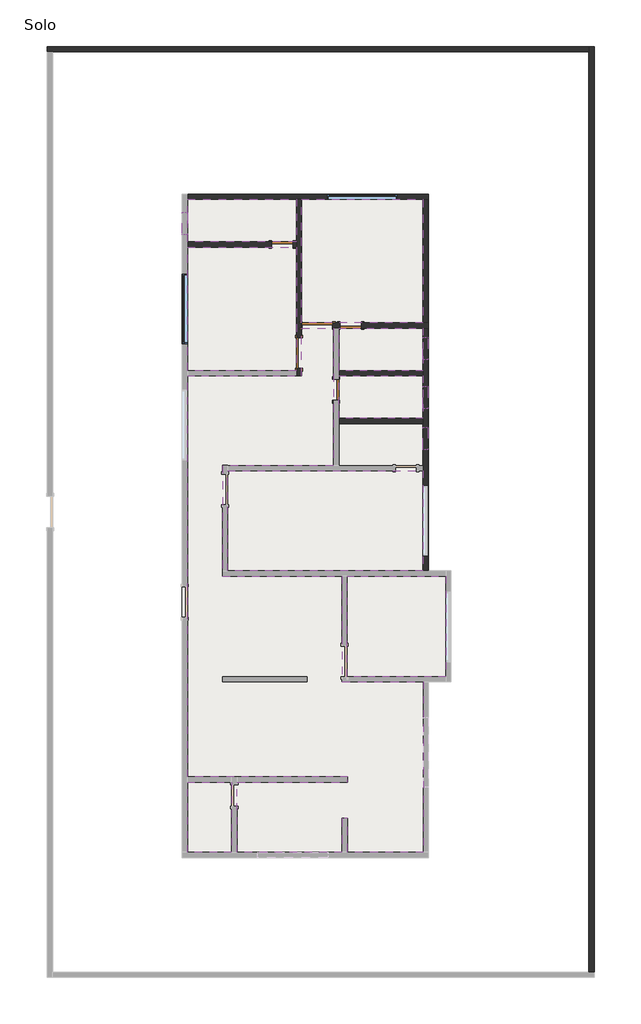
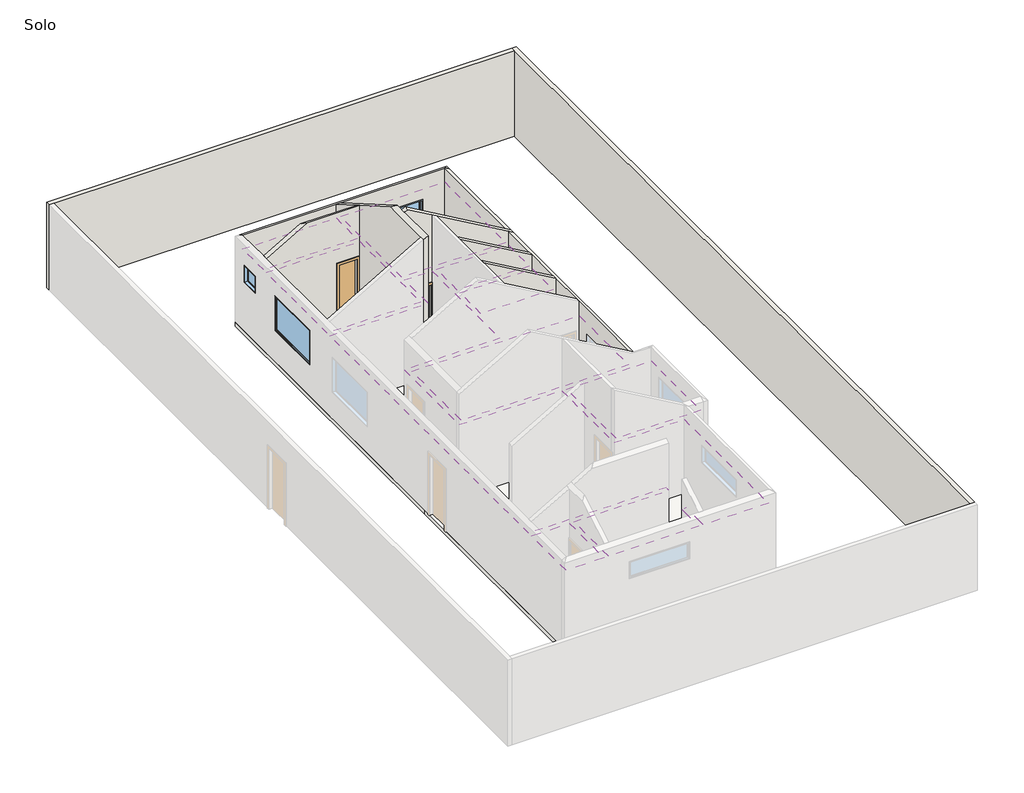
# One storey, part 2 of 2: 16 coverings, 9 walls, 6 windows, 5 doors, 1 slab.
"""IFC4 building model written with IfcOpenShell, lengths in millimetres."""

import ifcopenshell
import ifcopenshell.guid

model = None  # the IFC model being written
_history = None  # IfcOwnerHistory: only IFC2X3 demands one
_inside = {}  # id of a spatial element -> (the spatial element, [elements in it])
_under = {}  # id of a project, library or spatial element -> (it, [spatial elements below it])
_declared = {}  # id of a project -> (the project, [libraries it declares])
_typed = {}  # id of a type object -> (the type object, [elements of that type])
_made_of = {}  # id of a material, layer set ... -> (it, [elements and type objects made of it])


def new_model(schema):
    """Start an empty IFC model of exactly this schema.

    Asked for "IFC4X3", IfcOpenShell would pick the latest addendum, in which some entities
    have other attributes; the version numbers below select the first issue.
    IFC2X3 requires an IfcOwnerHistory on every rooted entity: one is made here for all.
    """
    global model, _history
    if schema == "IFC4X3":
        model = ifcopenshell.file(schema_version=(4, 3, 0, 0))
    else:
        model = ifcopenshell.file(schema=schema)
    _inside.clear()
    _under.clear()
    _declared.clear()
    _typed.clear()
    _made_of.clear()
    _history = None
    if model.schema == "IFC2X3":
        org = make("IfcOrganization", Name="unknown")
        user = make(
            "IfcPersonAndOrganization",
            ThePerson=make("IfcPerson", FamilyName="unknown"),
            TheOrganization=org,
        )
        app = make(
            "IfcApplication",
            ApplicationDeveloper=org,
            Version="unknown",
            ApplicationFullName="unknown",
            ApplicationIdentifier="unknown",
        )
        _history = make(
            "IfcOwnerHistory",
            OwningUser=user,
            OwningApplication=app,
            ChangeAction="ADDED",
            CreationDate=0,
        )
    return model


def make(cls, **values):
    """One entity of the class cls with the attributes given. An attribute that is None is left unset."""
    return model.create_entity(
        cls, **{name: value for name, value in values.items() if value is not None}
    )


def rooted(cls, **values):
    """An entity with a GlobalId (a new one), such as an element, a storey or a relation."""
    return make(cls, GlobalId=ifcopenshell.guid.new(), OwnerHistory=_history, **values)


def si_unit(unit_type, name, prefix=None):
    """IfcSIUnit, for example si_unit("LENGTHUNIT", "METRE", prefix="MILLI")."""
    return make("IfcSIUnit", UnitType=unit_type, Prefix=prefix, Name=name)


def assignment(units):
    """IfcUnitAssignment: the units of a project."""
    return None if units is None else make("IfcUnitAssignment", Units=units)


def point(xyz):
    """IfcCartesianPoint."""
    return None if xyz is None else make("IfcCartesianPoint", Coordinates=xyz)


def direction(xyz):
    """IfcDirection."""
    return None if xyz is None else make("IfcDirection", DirectionRatios=xyz)


def frame(location, z_axis=None, x_axis=None):
    """IfcAxis2Placement3D, a coordinate frame: its origin and axes. An axis left out is left unset."""
    return make(
        "IfcAxis2Placement3D",
        Location=point(location),
        Axis=direction(z_axis),
        RefDirection=direction(x_axis),
    )


def origin():
    """The frame at (0, 0, 0) with its axes left unset."""
    return frame((0.0, 0.0, 0.0))


def origin_with_axes():
    """The frame at (0, 0, 0) with the z axis (0, 0, 1) and the x axis (1, 0, 0) written out."""
    return frame((0.0, 0.0, 0.0), z_axis=(0.0, 0.0, 1.0), x_axis=(1.0, 0.0, 0.0))


def place(relative_to, where):
    """IfcLocalPlacement: puts the frame where relative to a parent placement (None: the world)."""
    return make(
        "IfcLocalPlacement", PlacementRelTo=relative_to, RelativePlacement=where
    )


def context(
    kind, dimensions, precision=None, world=None, true_north=None, identifier=None
):
    """IfcGeometricRepresentationContext, for example the 3D "Model" context."""
    return make(
        "IfcGeometricRepresentationContext",
        ContextIdentifier=identifier,
        ContextType=kind,
        CoordinateSpaceDimension=dimensions,
        Precision=precision,
        WorldCoordinateSystem=world,
        TrueNorth=true_north,
    )


def project(units=None, contexts=None):
    """IfcProject with its units and contexts."""
    return rooted(
        "IfcProject",
        Name="project",
        RepresentationContexts=contexts,
        UnitsInContext=assignment(units),
    )


def spatial(cls, under=None, at=None, **own):
    """A site, building, storey or space (cls), placed at a placement, below another one or the project."""
    s = rooted(cls, ObjectPlacement=at, **own)
    if under is not None:
        _under.setdefault(under.id(), (under, []))[1].append(s)
    return s


def polyline(points):
    """IfcPolyline through the points."""
    return make("IfcPolyline", Points=[point(p) for p in points])


def outline(outer, holes=None, kind="AREA"):
    """IfcArbitraryClosedProfileDef: a profile drawn as a closed curve; with holes, ...WithVoids."""
    if holes is None:
        return make("IfcArbitraryClosedProfileDef", ProfileType=kind, OuterCurve=outer)
    return make(
        "IfcArbitraryProfileDefWithVoids",
        ProfileType=kind,
        OuterCurve=outer,
        InnerCurves=holes,
    )


def extrude(swept, where, along, depth):
    """IfcExtrudedAreaSolid: the profile swept, set in the frame where, extruded along a direction by depth."""
    return make(
        "IfcExtrudedAreaSolid",
        SweptArea=swept,
        Position=where,
        ExtrudedDirection=direction(along),
        Depth=depth,
    )


def faces_of(points, faces, orient=None, outer=None):
    """IfcFace entities. A face is a list of loops; a loop is a list of indices into points, from 0.

    orient and outer hold one flag for each loop. By default every Orientation is true, the
    first loop of a face is its IfcFaceOuterBound and the others are IfcFaceBound.
    """
    made = []
    for i, loops in enumerate(faces):
        bounds = []
        for j, loop in enumerate(loops):
            is_outer = j == 0 if outer is None else outer[i][j]
            bounds.append(
                make(
                    "IfcFaceOuterBound" if is_outer else "IfcFaceBound",
                    Bound=make("IfcPolyLoop", Polygon=[points[k] for k in loop]),
                    Orientation=True if orient is None else orient[i][j],
                )
            )
        made.append(make("IfcFace", Bounds=bounds))
    return made


def faceted_brep(points, faces, orient=None, outer=None, voids=None):
    """IfcFacetedBrep: a solid bounded by flat faces; with voids (closed shells), ...WithVoids."""
    shared = [point(p) for p in points]
    hull = make("IfcClosedShell", CfsFaces=faces_of(shared, faces, orient, outer))
    if voids is None:
        return make("IfcFacetedBrep", Outer=hull)
    return make(
        "IfcFacetedBrepWithVoids",
        Outer=hull,
        Voids=[
            make(cls, CfsFaces=faces_of(shared, fs, o, b)) for cls, fs, o, b in voids
        ],
    )


def shape(context_of_items, identifier, shape_type, items):
    """IfcShapeRepresentation: the items that make up one representation, for example the "Body"."""
    return make(
        "IfcShapeRepresentation",
        ContextOfItems=context_of_items,
        RepresentationIdentifier=identifier,
        RepresentationType=shape_type,
        Items=items,
    )


def source(mapping_origin, context_of_items, identifier, shape_type, items):
    """IfcRepresentationMap: a shape defined once, which mapped items show again and again."""
    return make(
        "IfcRepresentationMap",
        MappingOrigin=mapping_origin,
        MappedRepresentation=shape(context_of_items, identifier, shape_type, items),
    )


def transform(
    local_origin,
    x_axis=None,
    y_axis=None,
    z_axis=None,
    scale=None,
    scale2=None,
    scale3=None,
    uniform=True,
):
    """IfcCartesianTransformationOperator3D, or its non-uniform kind. x_axis, y_axis, z_axis: its Axis1, 2, 3."""
    if uniform:
        return make(
            "IfcCartesianTransformationOperator3D",
            Axis1=direction(x_axis),
            Axis2=direction(y_axis),
            LocalOrigin=point(local_origin),
            Scale=scale,
            Axis3=direction(z_axis),
        )
    return make(
        "IfcCartesianTransformationOperator3DnonUniform",
        Axis1=direction(x_axis),
        Axis2=direction(y_axis),
        LocalOrigin=point(local_origin),
        Scale=scale,
        Axis3=direction(z_axis),
        Scale2=scale2,
        Scale3=scale3,
    )


def mapped(mapping_source, mapping_target):
    """IfcMappedItem: shows the shape of a source again, moved by a transform."""
    return make(
        "IfcMappedItem", MappingSource=mapping_source, MappingTarget=mapping_target
    )


def made_of(thing, what):
    """Note that an element or type object is made of a material, layer set ...; save() writes the relation."""
    if what is not None:
        _made_of.setdefault(what.id(), (what, []))[1].append(thing)
    return thing


def element(
    cls,
    number,
    at=None,
    inside=None,
    cuts=None,
    type_object=None,
    material=None,
    context=None,
    identifier="Body",
    shape_type=None,
    held_by="IfcProductDefinitionShape",
    body=None,
    shapes=None,
    **own,
):
    """One element of the class cls, such as IfcWall. Its Tag is "e" and its number.

    at: its placement. inside: the storey or other place that contains it. cuts: it is an
    opening in that element (IfcRelVoidsElement). A single representation is given by context,
    identifier, shape_type and body (its items); several are given by shapes. held_by: the class
    of the entity that holds the representations. save() writes the other relations.
    """
    e = rooted(cls, Tag="e%d" % number, ObjectPlacement=at, **own)
    if body is not None:
        shapes = [shape(context, identifier, shape_type, body)]
    if shapes is not None:
        e.Representation = make(held_by, Representations=shapes)
    if inside is not None:
        _inside.setdefault(inside.id(), (inside, []))[1].append(e)
    if cuts is not None:
        rooted(
            "IfcRelVoidsElement", RelatingBuildingElement=cuts, RelatedOpeningElement=e
        )
    if type_object is not None:
        _typed.setdefault(type_object.id(), (type_object, []))[1].append(e)
    return made_of(e, material)


def aggregate(whole, parts):
    """IfcRelAggregates: a whole, such as a stair, and the parts it consists of."""
    return rooted("IfcRelAggregates", RelatingObject=whole, RelatedObjects=parts)


def save(model, path):
    """Write the relations noted so far, then the file.

    IfcRelAggregates (storeys below a building ...), IfcRelContainedInSpatialStructure (elements
    in a storey), IfcRelDefinesByType, IfcRelAssociatesMaterial and IfcRelDeclares: one each for
    every whole, place, type object, material and project.
    """
    for whole, parts in _under.values():
        aggregate(whole, parts)
    for where, things in _inside.values():
        rooted(
            "IfcRelContainedInSpatialStructure",
            RelatedElements=things,
            RelatingStructure=where,
        )
    for kind, things in _typed.values():
        rooted("IfcRelDefinesByType", RelatedObjects=things, RelatingType=kind)
    for what, things in _made_of.values():
        rooted("IfcRelAssociatesMaterial", RelatedObjects=things, RelatingMaterial=what)
    for by, libraries in _declared.values():
        rooted("IfcRelDeclares", RelatingContext=by, RelatedDefinitions=libraries)
    model.write(path)


def door_0762_x_2032mm_f712f77f(model_context):
    return source(origin(), model_context, "Body", "SweptSolid", [
        extrude(outline(polyline([(2108.0, -376.0), (0.0, -376.0), (0.0, -300.0), (2032.0, -300.0), (2032.0, 300.0), (0.0, 300.0), (0.0, 376.0), (2108.0, 376.0), (2108.0, -376.0)])), frame((0.0, 75.0, 0.0), z_axis=(0.0, 1.0, 0.0), x_axis=(0.0, 0.0, 1.0)), (0.0, 0.0, 1.0), 25.0),
        extrude(outline(polyline([(2108.0, 376.0), (2108.0, -376.0), (0.0, -376.0), (0.0, -300.0), (2032.0, -300.0), (2032.0, 300.0), (0.0, 300.0), (0.0, 376.0), (2108.0, 376.0)])), frame((0.0, -100.0, 0.0), z_axis=(0.0, 1.0, 0.0), x_axis=(0.0, 0.0, 1.0)), (0.0, 0.0, 1.0), 25.0),
        extrude(outline(polyline([(300.0, 24.0), (-300.0, 24.0), (-300.0, 75.0), (300.0, 75.0), (300.0, 24.0)])), origin_with_axes(), (0.0, 0.0, 1.0), 2032.0),
    ])


def door_0762_x_2032mm_24b9c1ed(model_context):
    return source(origin(), model_context, "Body", "SweptSolid", [
        extrude(outline(polyline([(2108.0, -376.0), (0.0, -376.0), (0.0, -300.0), (2032.0, -300.0), (2032.0, 300.0), (0.0, 300.0), (0.0, 376.0), (2108.0, 376.0), (2108.0, -376.0)])), frame((0.0, -100.0, 0.0), z_axis=(0.0, 1.0, 0.0), x_axis=(0.0, 0.0, 1.0)), (0.0, 0.0, 1.0), 25.0),
        extrude(outline(polyline([(2108.0, 376.0), (2108.0, -376.0), (0.0, -376.0), (0.0, -300.0), (2032.0, -300.0), (2032.0, 300.0), (0.0, 300.0), (0.0, 376.0), (2108.0, 376.0)])), frame((0.0, 75.0, 0.0), z_axis=(0.0, 1.0, 0.0), x_axis=(0.0, 0.0, 1.0)), (0.0, 0.0, 1.0), 25.0),
        extrude(outline(polyline([(300.0, -24.0), (300.0, -75.0), (-300.0, -75.0), (-300.0, -24.0), (300.0, -24.0)])), origin_with_axes(), (0.0, 0.0, 1.0), 2032.0),
    ])


def door_0864_x_2134mm_0748c0c9(model_context):
    return source(origin(), model_context, "Body", "SweptSolid", [
        extrude(outline(polyline([(2210.0, -508.0), (0.0, -508.0), (0.0, -432.0), (2134.0, -432.0), (2134.0, 432.0), (0.0, 432.0), (0.0, 508.0), (2210.0, 508.0), (2210.0, -508.0)])), frame((0.0, -100.0, 0.0), z_axis=(0.0, 1.0, 0.0), x_axis=(0.0, 0.0, 1.0)), (0.0, 0.0, 1.0), 25.0),
        extrude(outline(polyline([(2210.0, 508.0), (2210.0, -508.0), (0.0, -508.0), (0.0, -432.0), (2134.0, -432.0), (2134.0, 432.0), (0.0, 432.0), (0.0, 508.0), (2210.0, 508.0)])), frame((0.0, 75.0, 0.0), z_axis=(0.0, 1.0, 0.0), x_axis=(0.0, 0.0, 1.0)), (0.0, 0.0, 1.0), 25.0),
        extrude(outline(polyline([(432.0, -24.0), (432.0, -75.0), (-432.0, -75.0), (-432.0, -24.0), (432.0, -24.0)])), origin_with_axes(), (0.0, 0.0, 1.0), 2134.0),
    ])


def m_fixo_0610_x_1830mm_9119c720(model_context):
    return source(origin(), model_context, "Body", "SweptSolid", [
        extrude(outline(polyline([(-257.0, 53.0), (257.0, 53.0), (257.0, 41.0), (-257.0, 41.0), (-257.0, 53.0)])), frame((0.0, 0.0, 668.0), z_axis=(0.0, 0.0, 1.0), x_axis=(1.0, 0.0, 0.0)), (0.0, 0.0, 1.0), 474.0),
        extrude(outline(polyline([(1186.0, -301.0), (624.0, -301.0), (624.0, 301.0), (1186.0, 301.0), (1186.0, -301.0)]), holes=[polyline([(1142.0, -257.0), (1142.0, 257.0), (668.0, 257.0), (668.0, -257.0), (1142.0, -257.0)])]), frame((0.0, 25.0, 0.0), z_axis=(0.0, 1.0, 0.0), x_axis=(0.0, 0.0, 1.0)), (0.0, 0.0, 1.0), 44.0),
        extrude(outline(polyline([(1205.0, -320.0), (605.0, -320.0), (605.0, 320.0), (1205.0, 320.0), (1205.0, -320.0)]), holes=[polyline([(1186.0, -301.0), (1186.0, 301.0), (624.0, 301.0), (624.0, -301.0), (1186.0, -301.0)])]), frame((0.0, 25.0, 0.0), z_axis=(0.0, 1.0, 0.0), x_axis=(0.0, 0.0, 1.0)), (0.0, 0.0, 1.0), 63.0),
        extrude(outline(polyline([(1205.0, -320.0), (605.0, -320.0), (605.0, 320.0), (1205.0, 320.0), (1205.0, -320.0)]), holes=[polyline([(1173.0, -288.0), (1173.0, 288.0), (637.0, 288.0), (637.0, -288.0), (1173.0, -288.0)])]), frame((0.0, -62.0, 0.0), z_axis=(0.0, 1.0, 0.0), x_axis=(0.0, 0.0, 1.0)), (0.0, 0.0, 1.0), 87.0),
    ])


def m_fixo_0915_x_1220mm_8e554ddc(model_context):
    return source(origin(), model_context, "Body", "SweptSolid", [
        extrude(outline(polyline([(-937.0, 53.0), (937.0, 53.0), (937.0, 41.0), (-937.0, 41.0), (-937.0, 53.0)])), frame((0.0, 0.0, 978.0), z_axis=(0.0, 0.0, 1.0), x_axis=(1.0, 0.0, 0.0)), (0.0, 0.0, 1.0), 1094.0),
        extrude(outline(polyline([(2116.0, -981.0), (934.0, -981.0), (934.0, 981.0), (2116.0, 981.0), (2116.0, -981.0)]), holes=[polyline([(2072.0, -937.0), (2072.0, 937.0), (978.0, 937.0), (978.0, -937.0), (2072.0, -937.0)])]), frame((0.0, 25.0, 0.0), z_axis=(0.0, 1.0, 0.0), x_axis=(0.0, 0.0, 1.0)), (0.0, 0.0, 1.0), 44.0),
        extrude(outline(polyline([(2135.0, -1000.0), (915.0, -1000.0), (915.0, 1000.0), (2135.0, 1000.0), (2135.0, -1000.0)]), holes=[polyline([(2116.0, -981.0), (2116.0, 981.0), (934.0, 981.0), (934.0, -981.0), (2116.0, -981.0)])]), frame((0.0, 25.0, 0.0), z_axis=(0.0, 1.0, 0.0), x_axis=(0.0, 0.0, 1.0)), (0.0, 0.0, 1.0), 63.0),
        extrude(outline(polyline([(2135.0, -1000.0), (915.0, -1000.0), (915.0, 1000.0), (2135.0, 1000.0), (2135.0, -1000.0)]), holes=[polyline([(2103.0, -968.0), (2103.0, 968.0), (947.0, 968.0), (947.0, -968.0), (2103.0, -968.0)])]), frame((0.0, -62.0, 0.0), z_axis=(0.0, 1.0, 0.0), x_axis=(0.0, 0.0, 1.0)), (0.0, 0.0, 1.0), 87.0),
    ])


model = new_model("IFC4")

# Units and contexts
model_context = context("Model", 3, world=origin())
ifc_project = project(units=[si_unit("LENGTHUNIT", "METRE", prefix="MILLI")], contexts=[model_context])

# Site, building, storey
site = spatial("IfcSite", under=ifc_project)
building = spatial("IfcBuilding", under=site)
storey = spatial("IfcBuildingStorey", under=building, Name="Solo", Elevation=0.0)

# Coverings
placement = place(None, origin())
element("IfcCovering", 1, ObjectType="Simples", at=placement, inside=storey, context=model_context, shape_type="SweptSolid", body=[
    extrude(outline(polyline([(-6285.8698767, 7725.0972586), (-6285.8698767, 8932.5972586), (-3187.4041224, 8932.5972586), (-3187.4041224, 7725.0972586), (-6285.8698767, 7725.0972586)])), frame((0.0, 0.0, 2600.0), z_axis=(0.0, 0.0, 1.0), x_axis=(1.0, 0.0, 0.0)), (0.0, 0.0, 1.0), 57.0),
])
element("IfcCovering", 2, ObjectType="Simples", at=placement, inside=storey, context=model_context, shape_type="SweptSolid", body=[
    extrude(outline(polyline([(-6285.8698767, 7725.0972586), (-6285.8698767, 8932.5972586), (-3187.4041224, 8932.5972586), (-3187.4041224, 7725.0972586), (-6285.8698767, 7725.0972586)])), frame((0.0, 0.0, 2600.0), z_axis=(0.0, 0.0, 1.0), x_axis=(1.0, 0.0, 0.0)), (0.0, 0.0, 1.0), 57.0),
])
element("IfcCovering", 3, ObjectType="Simples", at=placement, inside=storey, context=model_context, shape_type="SweptSolid", body=[
    extrude(outline(polyline([(-6285.8698767, 4070.0972586), (-6285.8698767, 7575.0972586), (-3187.4041224, 7575.0972586), (-3187.4041224, 4070.0972586), (-6285.8698767, 4070.0972586)])), frame((0.0, 0.0, 2600.0), z_axis=(0.0, 0.0, 1.0), x_axis=(1.0, 0.0, 0.0)), (0.0, 0.0, 1.0), 57.0),
])
element("IfcCovering", 4, ObjectType="Simples", at=placement, inside=storey, context=model_context, shape_type="SweptSolid", body=[
    extrude(outline(polyline([(-6285.8698767, 4070.0972586), (-6285.8698767, 7575.0972586), (-3187.4041224, 7575.0972586), (-3187.4041224, 4070.0972586), (-6285.8698767, 4070.0972586)])), frame((0.0, 0.0, 2600.0), z_axis=(0.0, 0.0, 1.0), x_axis=(1.0, 0.0, 0.0)), (0.0, 0.0, 1.0), 57.0),
])
element("IfcCovering", 5, ObjectType="Simples", at=placement, inside=storey, context=model_context, shape_type="SweptSolid", body=[
    extrude(outline(polyline([(-3037.4041224, 8932.5972586), (409.1301231, 8932.5972586), (409.1301231, 5423.5630139), (-3037.4041224, 5423.5630139), (-3037.4041224, 8932.5972586)])), frame((0.0, 0.0, 2600.0), z_axis=(0.0, 0.0, 1.0), x_axis=(1.0, 0.0, 0.0)), (0.0, 0.0, 1.0), 57.0),
])
element("IfcCovering", 6, ObjectType="Simples", at=placement, inside=storey, context=model_context, shape_type="SweptSolid", body=[
    extrude(outline(polyline([(-6285.8698767, 7725.0972586), (-6285.8698767, 8932.5972586), (-3187.4041224, 8932.5972586), (-3187.4041224, 7725.0972586), (-6285.8698767, 7725.0972586)])), frame((0.0, 0.0, 2600.0), z_axis=(0.0, 0.0, 1.0), x_axis=(1.0, 0.0, 0.0)), (0.0, 0.0, 1.0), 57.0),
])
element("IfcCovering", 7, ObjectType="Simples", at=placement, inside=storey, context=model_context, shape_type="SweptSolid", body=[
    extrude(outline(polyline([(-6285.8698767, 4070.0972586), (-6285.8698767, 7575.0972586), (-3187.4041224, 7575.0972586), (-3187.4041224, 4070.0972586), (-6285.8698767, 4070.0972586)])), frame((0.0, 0.0, 2600.0), z_axis=(0.0, 0.0, 1.0), x_axis=(1.0, 0.0, 0.0)), (0.0, 0.0, 1.0), 57.0),
])
element("IfcCovering", 8, ObjectType="Simples", at=placement, inside=storey, context=model_context, shape_type="SweptSolid", body=[
    extrude(outline(polyline([(-6285.8698767, 4070.0972586), (-6285.8698767, 7575.0972586), (-3187.4041224, 7575.0972586), (-3187.4041224, 4070.0972586), (-6285.8698767, 4070.0972586)])), frame((0.0, 0.0, 2600.0), z_axis=(0.0, 0.0, 1.0), x_axis=(1.0, 0.0, 0.0)), (0.0, 0.0, 1.0), 57.0),
])
element("IfcCovering", 9, ObjectType="Simples", at=placement, inside=storey, context=model_context, shape_type="SweptSolid", body=[
    extrude(outline(polyline([(-3037.4041224, 8932.5972586), (409.1301231, 8932.5972586), (409.1301231, 5423.5630139), (-3037.4041224, 5423.5630139), (-3037.4041224, 8932.5972586)])), frame((0.0, 0.0, 2600.0), z_axis=(0.0, 0.0, 1.0), x_axis=(1.0, 0.0, 0.0)), (0.0, 0.0, 1.0), 57.0),
])
element("IfcCovering", 10, ObjectType="Simples", at=placement, inside=storey, context=model_context, shape_type="SweptSolid", body=[
    extrude(outline(polyline([(-1979.4742231, 5273.5630139), (409.1301231, 5273.5630139), (409.1301231, 4070.0972586), (-1979.4742231, 4070.0972586), (-1979.4742231, 5273.5630139)])), frame((0.0, 0.0, 2600.0), z_axis=(0.0, 0.0, 1.0), x_axis=(1.0, 0.0, 0.0)), (0.0, 0.0, 1.0), 57.0),
])
element("IfcCovering", 11, ObjectType="Simples", at=placement, inside=storey, context=model_context, shape_type="SweptSolid", body=[
    extrude(outline(polyline([(409.1301231, 3920.0972586), (409.1301231, 2713.9475745), (-1979.4742231, 2713.9475745), (-1979.4742231, 3920.0972586), (409.1301231, 3920.0972586)])), frame((0.0, 0.0, 2600.0), z_axis=(0.0, 0.0, 1.0), x_axis=(1.0, 0.0, 0.0)), (0.0, 0.0, 1.0), 57.0),
])
element("IfcCovering", 12, ObjectType="Simples", at=placement, inside=storey, context=model_context, shape_type="SweptSolid", body=[
    extrude(outline(polyline([(424.1301232, -9623.7945276), (-1735.8698771, -9623.7945276), (-1735.8698771, -8644.9027402), (-1885.8698771, -8644.9027402), (-1885.8698771, -9623.7945276), (-4875.9149651, -9623.7945276), (-4875.9149651, -7626.6262329), (-1735.8698771, -7626.6262329), (-1735.8698771, -7476.6262329), (-4950.9149651, -7476.6262329), (-6285.8698767, -7476.6262329), (-6285.8698767, 3920.0972586), (-3037.4041224, 3920.0972586), (-3037.4041224, 5273.5630139), (-2129.4742231, 5273.5630139), (-2129.4742231, 1370.0972582), (-5289.335632, 1370.0972582), (-5289.335632, -1774.902741), (-1895.8247891, -1774.902741), (-1895.8247891, -4774.9027402), (424.1301232, -4774.9027402), (424.1301232, -9623.7945276)]), holes=[polyline([(-2885.8698771, -4774.9027402), (-2885.8698771, -4624.9027402), (-5285.8698771, -4624.9027402), (-5285.8698771, -4774.9027402), (-2885.8698771, -4774.9027402)])]), frame((0.0, 0.0, 2600.0), z_axis=(0.0, 0.0, 1.0), x_axis=(1.0, 0.0, 0.0)), (0.0, 0.0, 1.0), 57.0),
])
element("IfcCovering", 13, ObjectType="Simples", at=placement, inside=storey, context=model_context, shape_type="SweptSolid", body=[
    extrude(outline(polyline([(409.1301231, 1220.0972582), (409.1301231, -1624.902741), (-5139.335632, -1624.902741), (-5139.335632, 1220.0972582), (409.1301231, 1220.0972582)])), frame((0.0, 0.0, 2600.0), z_axis=(0.0, 0.0, 1.0), x_axis=(1.0, 0.0, 0.0)), (0.0, 0.0, 1.0), 57.0),
])
element("IfcCovering", 14, ObjectType="Simples", at=placement, inside=storey, context=model_context, shape_type="SweptSolid", body=[
    extrude(outline(polyline([(-1745.8247891, -1774.902741), (1059.1301231, -1774.902741), (1059.1301231, -4624.9027402), (-1745.8247891, -4624.9027402), (-1745.8247891, -1774.902741)])), frame((0.0, 0.0, 2600.0), z_axis=(0.0, 0.0, 1.0), x_axis=(1.0, 0.0, 0.0)), (0.0, 0.0, 1.0), 57.0),
])
element("IfcCovering", 15, ObjectType="Simples", at=placement, inside=storey, context=model_context, shape_type="SweptSolid", body=[
    extrude(outline(polyline([(424.1301232, -9623.7945276), (-1735.8698771, -9623.7945276), (-1735.8698771, -8644.9027402), (-1885.8698771, -8644.9027402), (-1885.8698771, -9623.7945276), (-4875.9149651, -9623.7945276), (-4875.9149651, -7626.6262329), (-1735.8698771, -7626.6262329), (-1735.8698771, -7476.6262329), (-4950.9149651, -7476.6262329), (-6285.8698767, -7476.6262329), (-6285.8698767, 3920.0972586), (-3037.4041224, 3920.0972586), (-3037.4041224, 5273.5630139), (-2129.4742231, 5273.5630139), (-2129.4742231, 1370.0972582), (-5289.335632, 1370.0972582), (-5289.335632, -1774.902741), (-1895.8247891, -1774.902741), (-1895.8247891, -4774.9027402), (424.1301232, -4774.9027402), (424.1301232, -9623.7945276)]), holes=[polyline([(-2885.8698771, -4774.9027402), (-2885.8698771, -4624.9027402), (-5285.8698771, -4624.9027402), (-5285.8698771, -4774.9027402), (-2885.8698771, -4774.9027402)])]), frame((0.0, 0.0, 2600.0), z_axis=(0.0, 0.0, 1.0), x_axis=(1.0, 0.0, 0.0)), (0.0, 0.0, 1.0), 57.0),
])
element("IfcCovering", 16, ObjectType="Simples", at=placement, inside=storey, context=model_context, shape_type="SweptSolid", body=[
    extrude(outline(polyline([(-5025.9149651, -9623.7945276), (-6285.8698767, -9623.7945276), (-6285.8698767, -7626.6262329), (-5025.9149651, -7626.6262329), (-5025.9149651, -9623.7945276)])), frame((0.0, 0.0, 2600.0), z_axis=(0.0, 0.0, 1.0), x_axis=(1.0, 0.0, 0.0)), (0.0, 0.0, 1.0), 57.0),
])

# Doors
door_0762_x_2032mm_shape = door_0762_x_2032mm_f712f77f(model_context)
element("IfcDoor", 17, ObjectType="M_Folha única : 0762 x 2032mm", at=placement, inside=storey, context=model_context, shape_type="MappedRepresentation", body=[
    mapped(door_0762_x_2032mm_shape, transform((-3587.4041224, 7650.0972586, 0.0), x_axis=(1.0, 0.0, 0.0), y_axis=(0.0, 1.0, 0.0), z_axis=(0.0, 0.0, 1.0))),
])
element("IfcDoor", 18, ObjectType="M_Folha única : 0762 x 2032mm", at=placement, inside=storey, context=model_context, shape_type="MappedRepresentation", body=[
    mapped(door_0762_x_2032mm_shape, transform((-1639.4742231, 5348.5630139, 0.0), x_axis=(-1.0, 0.0, 0.0), y_axis=(0.0, -1.0, 0.0), z_axis=(0.0, 0.0, 1.0))),
])
door_0762_x_2032mm_2_shape = door_0762_x_2032mm_24b9c1ed(model_context)
element("IfcDoor", 19, ObjectType="M_Folha única : 0762 x 2032mm", at=placement, inside=storey, context=model_context, shape_type="MappedRepresentation", body=[
    mapped(door_0762_x_2032mm_2_shape, transform((-2054.4742231, 3520.0972586, 0.0), x_axis=(0.0, 1.0, 0.0), y_axis=(-1.0, 0.0, 0.0), z_axis=(0.0, 0.0, 1.0))),
])
door_0864_x_2134mm_shape = door_0864_x_2134mm_0748c0c9(model_context)
element("IfcDoor", 20, ObjectType="M_Folha única : 0864 x 2134mm", at=placement, inside=storey, context=model_context, shape_type="MappedRepresentation", body=[
    mapped(door_0864_x_2134mm_shape, transform((-3112.4041224, 4562.0972586, 0.0), x_axis=(0.0, -1.0, 0.0), y_axis=(1.0, 0.0, 0.0), z_axis=(0.0, 0.0, 1.0))),
])
element("IfcDoor", 21, ObjectType="M_Folha única : 0864 x 2134mm", at=placement, inside=storey, context=model_context, shape_type="MappedRepresentation", body=[
    mapped(door_0864_x_2134mm_shape, transform((-2586.5671697, 5348.5630139, 0.0), x_axis=(-1.0, 0.0, 0.0), y_axis=(0.0, -1.0, 0.0), z_axis=(0.0, 0.0, 1.0))),
])

# Slab
element("IfcSlab", 22, ObjectType="Genérico 150 mm", at=placement, inside=storey, context=model_context, shape_type="SweptSolid", body=[
    extrude(outline(polyline([(-6435.8698767, 9082.5972586), (574.1301232, 9082.5972586), (574.1301232, -1624.902741), (1209.1301231, -1624.902741), (1209.1301231, -4774.9027402), (574.1301232, -4774.9027402), (574.1301232, -9773.7945276), (-6435.8698767, -9773.7945276), (-6435.8698767, -1774.902741), (-6435.8698767, 9082.5972586)])), frame((0.0, 0.0, -150.0), z_axis=(0.0, 0.0, 1.0), x_axis=(1.0, 0.0, 0.0)), (0.0, 0.0, 1.0), 150.0),
])

# Walls
element("IfcWall", 23, ObjectType="Genérico - 140 mm Alvenaria", at=placement, inside=storey, context=model_context, shape_type="Brep", body=[
    faceted_brep([(564.1301231, 9082.5972586, 0.0), (-6285.8698767, 9082.5972586, 0.0), (-6285.8698767, 9082.5972586, 3000.0), (564.1301231, 9082.5972586, 3000.0), (-2314.1369996, 9082.5972586, 1021.335877), (-314.1369996, 9082.5972586, 1021.335877), (-314.1369996, 9082.5972586, 2241.335877), (-2314.1369996, 9082.5972586, 2241.335877), (564.1301231, 8932.5972586, 0.0), (564.1301231, 8932.5972586, 3005.7735027), (559.1301231, 8932.5972586, 3008.6602541), (424.1301232, 8932.5972586, 3086.6025404), (409.1301231, 8932.5972586, 3086.6025404), (-3037.4041224, 8932.5972586, 3086.6025404), (-3187.4041224, 8932.5972586, 3086.6025404), (-6285.8698767, 8932.5972586, 3086.6025404), (-6285.8698767, 8932.5972586, 0.0), (-3187.4041224, 8932.5972586, 0.0), (-3037.4041224, 8932.5972586, 0.0), (409.1301231, 8932.5972586, 0.0), (559.1301231, 8932.5972586, 0.0), (-2314.1369996, 8932.5972586, 1021.335877), (-2314.1369996, 8932.5972586, 2241.335877), (-314.1369996, 8932.5972586, 2241.335877), (-314.1369996, 8932.5972586, 1021.335877), (564.1301231, 9072.5972586, 3005.7735027)], [[[0, 1, 2, 3], [4, 5, 6, 7]], [[8, 9, 10, 11, 12, 13, 14, 15, 16, 17, 18, 19, 20], [21, 22, 23, 24]], [[1, 0, 8, 20, 19, 18, 17, 16]], [[0, 3, 25, 9, 8]], [[2, 1, 16, 15]], [[22, 21, 4, 7]], [[23, 22, 7, 6]], [[24, 23, 6, 5]], [[21, 24, 5, 4]], [[3, 2, 15, 14, 13, 12, 11, 25]], [[11, 10, 9, 25]]]),
])
element("IfcWall", 24, ObjectType="Genérico - 140 mm Alvenaria", at=placement, inside=storey, context=model_context, shape_type="Brep", body=[
    faceted_brep([(-3187.4041224, 7725.0972586, 0.0), (-3287.4041224, 7725.0972586, 0.0), (-3287.4041224, 7725.0972586, 2032.0), (-3887.4041224, 7725.0972586, 2032.0), (-3887.4041224, 7725.0972586, 0.0), (-6285.8698767, 7725.0972586, 0.0), (-6285.8698767, 7725.0972586, 3086.6025404), (-5078.3698767, 7725.0972586, 3783.7529904), (-3187.4041224, 7725.0972586, 3783.7529904), (-3287.4041224, 7575.0972586, 2032.0), (-3287.4041224, 7575.0972586, 0.0), (-3187.4041224, 7575.0972586, 0.0), (-3187.4041224, 7575.0972586, 3870.3555308), (-4928.3698767, 7575.0972586, 3870.3555308), (-6285.8698767, 7575.0972586, 3086.6025404), (-6285.8698767, 7575.0972586, 0.0), (-3887.4041224, 7575.0972586, 0.0), (-3887.4041224, 7575.0972586, 2032.0)], [[[0, 1, 2, 3, 4, 5, 6, 7, 8]], [[9, 10, 11, 12, 13, 14, 15, 16, 17]], [[16, 15, 5, 4]], [[11, 10, 1, 0]], [[6, 5, 15, 14]], [[0, 8, 12, 11]], [[2, 1, 10, 9]], [[3, 2, 9, 17]], [[4, 3, 17, 16]], [[8, 7, 13, 12]], [[7, 6, 14, 13]]]),
])
element("IfcWall", 25, ObjectType="Genérico - 140 mm Alvenaria", at=placement, inside=storey, context=model_context, shape_type="Brep", body=[
    faceted_brep([(-3037.4041224, 3920.0972586, 0.0), (-3037.4041224, 4130.0972586, 0.0), (-3037.4041224, 4130.0972586, 2134.0), (-3037.4041224, 4994.0972586, 2134.0), (-3037.4041224, 4994.0972586, 0.0), (-3037.4041224, 5273.5630139, 0.0), (-3037.4041224, 5423.5630139, 0.0), (-3037.4041224, 8932.5972586, 0.0), (-3037.4041224, 8932.5972586, 3086.6025404), (-3037.4041224, 5684.1315043, 4962.1051181), (-3037.4041224, 5423.5630139, 4962.1051181), (-3037.4041224, 5273.5630139, 4962.1051181), (-3037.4041224, 3920.0972586, 4962.1051181), (-3187.4041224, 4130.0972586, 2134.0), (-3187.4041224, 4130.0972586, 0.0), (-3187.4041224, 4070.0972586, 0.0), (-3187.4041224, 3920.0972586, 0.0), (-3187.4041224, 3920.0972586, 4875.5025777), (-3187.4041224, 4070.0972586, 4875.5025777), (-3187.4041224, 5834.1315043, 4875.5025777), (-3187.4041224, 7575.0972586, 3870.3555308), (-3187.4041224, 7725.0972586, 3783.7529904), (-3187.4041224, 8932.5972586, 3086.6025404), (-3187.4041224, 8932.5972586, 0.0), (-3187.4041224, 7725.0972586, 0.0), (-3187.4041224, 7575.0972586, 0.0), (-3187.4041224, 4994.0972586, 0.0), (-3187.4041224, 4994.0972586, 2134.0)], [[[0, 1, 2, 3, 4, 5, 6, 7, 8, 9, 10, 11, 12]], [[13, 14, 15, 16, 17, 18, 19, 20, 21, 22, 23, 24, 25, 26, 27]], [[16, 15, 14, 1, 0]], [[26, 25, 24, 23, 7, 6, 5, 4]], [[8, 7, 23, 22]], [[0, 12, 17, 16]], [[2, 1, 14, 13]], [[3, 2, 13, 27]], [[4, 3, 27, 26]], [[12, 11, 10, 9, 19, 18, 17]], [[9, 8, 22, 21, 20, 19]]]),
])
element("IfcWall", 26, ObjectType="Genérico - 140 mm Alvenaria", at=placement, inside=storey, context=model_context, shape_type="Brep", body=[
    faceted_brep([(-1939.4742231, 5423.5630139, 2032.0), (-1939.4742231, 5423.5630139, 0.0), (-2154.5671697, 5423.5630139, 0.0), (-2154.5671697, 5423.5630139, 2134.0), (-3018.5671697, 5423.5630139, 2134.0), (-3018.5671697, 5423.5630139, 0.0), (-3037.4041224, 5423.5630139, 0.0), (-3037.4041224, 5423.5630139, 4962.1051181), (-2930.8698768, 5423.5630139, 5023.6126935), (564.1301231, 5423.5630139, 3005.7735027), (564.1301231, 5423.5630139, 0.0), (-1339.4742231, 5423.5630139, 0.0), (-1339.4742231, 5423.5630139, 2032.0), (-2154.5671697, 5273.5630139, 0.0), (-2129.4742231, 5273.5630139, 0.0), (-1979.4742231, 5273.5630139, 0.0), (-1939.4742231, 5273.5630139, 0.0), (-1939.4742231, 5273.5630139, 2032.0), (-1339.4742231, 5273.5630139, 2032.0), (-1339.4742231, 5273.5630139, 0.0), (564.1301231, 5273.5630139, 0.0), (564.1301231, 5273.5630139, 3005.7735027), (-1979.4742231, 5273.5630139, 4474.3241567), (-2129.4742231, 5273.5630139, 4560.9266971), (-2930.8698768, 5273.5630139, 5023.6126935), (-3037.4041224, 5273.5630139, 4962.1051181), (-3037.4041224, 5273.5630139, 0.0), (-3018.5671697, 5273.5630139, 0.0), (-3018.5671697, 5273.5630139, 2134.0), (-2154.5671697, 5273.5630139, 2134.0)], [[[0, 1, 2, 3, 4, 5, 6, 7, 8, 9, 10, 11, 12]], [[13, 14, 15, 16, 17, 18, 19, 20, 21, 22, 23, 24, 25, 26, 27, 28, 29]], [[6, 5, 27, 26]], [[11, 10, 20, 19]], [[2, 1, 16, 15, 14, 13]], [[10, 9, 21, 20]], [[7, 6, 26, 25]], [[28, 27, 5, 4]], [[29, 28, 4, 3]], [[13, 29, 3, 2]], [[17, 16, 1, 0]], [[18, 17, 0, 12]], [[19, 18, 12, 11]], [[9, 8, 24, 23, 22, 21]], [[8, 7, 25, 24]]]),
])
element("IfcWall", 27, ObjectType="Genérico - 140 mm Alvenaria", at=placement, inside=storey, context=model_context, shape_type="Brep", body=[
    faceted_brep([(409.1301231, 8932.5972586, 0.0), (409.1301231, 4070.0972586, 0.0), (409.1301231, 3920.0972586, 0.0), (409.1301231, 2713.9475745, 0.0), (409.1301231, 2563.9475745, 0.0), (409.1301231, 1370.0972582, 0.0), (409.1301231, 1220.0972582, 0.0), (409.1301231, -1624.902741, 0.0), (409.1301231, -1624.902741, 3095.2627944), (409.1301231, 1220.0972582, 3095.2627944), (409.1301231, 1370.0972582, 3095.2627944), (409.1301231, 2563.9475745, 3095.2627944), (409.1301231, 2713.9475745, 3095.2627944), (409.1301231, 3920.0972586, 3095.2627944), (409.1301231, 4070.0972586, 3095.2627944), (409.1301231, 8917.5972586, 3095.2627944), (409.1301231, 8932.5972586, 3086.6025404), (409.1301231, 2463.9475745, 1700.0), (409.1301231, 2463.9475745, 2300.0), (409.1301231, 1823.9475745, 2300.0), (409.1301231, 1823.9475745, 1700.0), (409.1301231, 2980.0972586, 1700.0), (409.1301231, 3620.0972586, 1700.0), (409.1301231, 3620.0972586, 2300.0), (409.1301231, 2980.0972586, 2300.0), (409.1301231, 4370.0972586, 1700.0), (409.1301231, 5010.0972586, 1700.0), (409.1301231, 5010.0972586, 2300.0), (409.1301231, 4370.0972586, 2300.0), (409.1301231, 800.0972582, 980.0), (409.1301231, 800.0972582, 2200.0), (409.1301231, -1199.9027418, 2200.0), (409.1301231, -1199.9027418, 980.0), (559.1301231, 8932.5972586, 0.0), (559.1301231, 8932.5972586, 3008.6602541), (559.1301231, -1624.902741, 3008.6602541), (559.1301231, -1624.902741, 0.0), (559.1301231, 2463.9475745, 1700.0), (559.1301231, 1823.9475745, 1700.0), (559.1301231, 1823.9475745, 2300.0), (559.1301231, 2463.9475745, 2300.0), (559.1301231, 2980.0972586, 1700.0), (559.1301231, 2980.0972586, 2300.0), (559.1301231, 3620.0972586, 2300.0), (559.1301231, 3620.0972586, 1700.0), (559.1301231, 4370.0972586, 1700.0), (559.1301231, 4370.0972586, 2300.0), (559.1301231, 5010.0972586, 2300.0), (559.1301231, 5010.0972586, 1700.0), (559.1301231, 800.0972582, 980.0), (559.1301231, -1199.9027418, 980.0), (559.1301231, -1199.9027418, 2200.0), (559.1301231, 800.0972582, 2200.0), (424.1301232, 8932.5972586, 3086.6025404)], [[[0, 1, 2, 3, 4, 5, 6, 7, 8, 9, 10, 11, 12, 13, 14, 15, 16], [17, 18, 19, 20], [21, 22, 23, 24], [25, 26, 27, 28], [29, 30, 31, 32]], [[33, 34, 35, 36], [37, 38, 39, 40], [41, 42, 43, 44], [45, 46, 47, 48], [49, 50, 51, 52]], [[7, 6, 5, 4, 3, 2, 1, 0, 33, 36]], [[0, 16, 53, 34, 33]], [[8, 7, 36, 35]], [[18, 17, 37, 40]], [[19, 18, 40, 39]], [[20, 19, 39, 38]], [[17, 20, 38, 37]], [[42, 41, 21, 24]], [[43, 42, 24, 23]], [[44, 43, 23, 22]], [[41, 44, 22, 21]], [[46, 45, 25, 28]], [[47, 46, 28, 27]], [[48, 47, 27, 26]], [[45, 48, 26, 25]], [[30, 29, 49, 52]], [[31, 30, 52, 51]], [[32, 31, 51, 50]], [[29, 32, 50, 49]], [[16, 15, 53]], [[15, 14, 13, 12, 11, 10, 9, 8, 35, 34, 53]]]),
])
element("IfcWall", 28, ObjectType="Genérico - 140 mm Alvenaria", at=placement, inside=storey, context=model_context, shape_type="SweptSolid", body=[
    extrude(outline(polyline([(0.0, -1979.4742231), (0.0, 409.1301231), (3095.2627944, 409.1301231), (4474.3241567, -1979.4742231), (0.0, -1979.4742231)])), frame((0.0, 2563.9475745, 0.0), z_axis=(0.0, 1.0, 0.0), x_axis=(0.0, 0.0, 1.0)), (0.0, 0.0, 1.0), 150.0),
])
element("IfcWall", 29, ObjectType="Genérico - 140 mm Alvenaria", at=placement, inside=storey, context=model_context, shape_type="SweptSolid", body=[
    extrude(outline(polyline([(0.0, -1979.4742231), (0.0, 409.1301231), (3095.2627944, 409.1301231), (4474.3241567, -1979.4742231), (0.0, -1979.4742231)])), frame((0.0, 3920.0972586, 0.0), z_axis=(0.0, 1.0, 0.0), x_axis=(0.0, 0.0, 1.0)), (0.0, 0.0, 1.0), 150.0),
])
element("IfcWall", 30, ObjectType="Genérico - 140 mm Alvenaria", at=placement, inside=storey, context=model_context, shape_type="Brep", body=[
    faceted_brep([(5284.1301231, -13024.9027402, 0.0), (5284.1301231, 13275.0972598, 0.0), (5284.1301231, 13275.0972598, 3000.0), (5284.1301231, -13024.9027402, 3000.0), (5134.1301231, -13024.9027402, 0.0), (5134.1301231, -13024.9027402, 3000.0), (5134.1301231, 13125.0972598, 3000.0), (5134.1301231, 13275.0972598, 3000.0), (5134.1301231, 13275.0972598, 0.0), (5134.1301231, 13125.0972598, 0.0)], [[[0, 1, 2, 3]], [[4, 5, 6, 7, 8, 9]], [[1, 0, 4, 9, 8]], [[3, 2, 7, 6, 5]], [[2, 1, 8, 7]], [[0, 3, 5, 4]]]),
])
element("IfcWall", 31, ObjectType="Genérico - 140 mm Alvenaria", at=placement, inside=storey, context=model_context, shape_type="Brep", body=[
    faceted_brep([(5134.1301231, 13275.0972598, 0.0), (-10265.8698769, 13275.0972598, 0.0), (-10265.8698769, 13275.0972598, 3000.0), (5134.1301231, 13275.0972598, 3000.0), (5134.1301231, 13125.0972598, 0.0), (5134.1301231, 13125.0972598, 3000.0), (-10115.8698769, 13125.0972598, 3000.0), (-10265.8698769, 13125.0972598, 3000.0), (-10265.8698769, 13125.0972598, 0.0), (-10115.8698769, 13125.0972598, 0.0)], [[[0, 1, 2, 3]], [[4, 5, 6, 7, 8, 9]], [[1, 0, 4, 9, 8]], [[3, 2, 7, 6, 5]], [[0, 3, 5, 4]], [[2, 1, 8, 7]]]),
])

# Windows
m_fixo_0610_x_1830mm_shape = m_fixo_0610_x_1830mm_9119c720(model_context)
element("IfcWindow", 32, ObjectType="M_Fixo : 0610 x 1830mm", at=placement, inside=storey, context=model_context, shape_type="MappedRepresentation", body=[
    mapped(m_fixo_0610_x_1830mm_shape, transform((471.1301231, 2143.9475745, 1095.0), x_axis=(0.0, -1.0, 0.0), y_axis=(1.0, 0.0, 0.0), z_axis=(0.0, 0.0, 1.0))),
])
element("IfcWindow", 33, ObjectType="M_Fixo : 0610 x 1830mm", at=placement, inside=storey, context=model_context, shape_type="MappedRepresentation", body=[
    mapped(m_fixo_0610_x_1830mm_shape, transform((497.1301231, 3300.0972586, 1095.0), x_axis=(0.0, 1.0, 0.0), y_axis=(-1.0, 0.0, 0.0), z_axis=(0.0, 0.0, 1.0))),
])
element("IfcWindow", 34, ObjectType="M_Fixo : 0610 x 1830mm", at=placement, inside=storey, context=model_context, shape_type="MappedRepresentation", body=[
    mapped(m_fixo_0610_x_1830mm_shape, transform((497.1301231, 4690.0972586, 1095.0), x_axis=(0.0, 1.0, 0.0), y_axis=(-1.0, 0.0, 0.0), z_axis=(0.0, 0.0, 1.0))),
])
element("IfcWindow", 35, ObjectType="M_Fixo : 0610 x 1830mm", at=placement, inside=storey, context=model_context, shape_type="MappedRepresentation", body=[
    mapped(m_fixo_0610_x_1830mm_shape, transform((-6373.8698767, 8252.5972586, 1095.0), x_axis=(0.0, -1.0, 0.0), y_axis=(1.0, 0.0, 0.0), z_axis=(0.0, 0.0, 1.0))),
])
m_fixo_0915_x_1220mm_shape = m_fixo_0915_x_1220mm_8e554ddc(model_context)
element("IfcWindow", 36, ObjectType="M_Fixo : 0915 x 1220mm", at=placement, inside=storey, context=model_context, shape_type="MappedRepresentation", body=[
    mapped(m_fixo_0915_x_1220mm_shape, transform((-1314.1369996, 8994.5972586, 106.335877), x_axis=(1.0, 0.0, 0.0), y_axis=(0.0, 1.0, 0.0), z_axis=(0.0, 0.0, 1.0))),
])
element("IfcWindow", 37, ObjectType="M_Fixo : 0915 x 1220mm", at=placement, inside=storey, context=model_context, shape_type="MappedRepresentation", body=[
    mapped(m_fixo_0915_x_1220mm_shape, transform((-6347.8698767, 5822.5972586, 165.5823766), x_axis=(0.0, 1.0, 0.0), y_axis=(-1.0, 0.0, 0.0), z_axis=(0.0, 0.0, 1.0))),
])

save(model, "model.ifc")

# Revit data of these elements
# Type "Simples"
#   built-in parameter 1002203 = 1 (stored number, unit not read)
#   built-in parameter 1002202 = 1 (stored number, unit not read)
#   Layers, outside or top first: 0.045 m "Camada de suporte de metal" (function 1); 0.012 m "Placa de gesso de parede" (function 1)
# Type "M_Folha única : 0762 x 2032mm"
#   Type Mark = "28"
#   Construction Type Id = "MDOOR"
#   Analytic Construction = "Metal"
#   Thickness = 0.051 m
#   Thermal Resistance (R) = 0.270117 (m²·K)/W
#   Heat Transfer Coefficient (U) = 3.7021 W/(m²·K)
#   Height = 2.032 m
#   Projeção da apara externa = 0.025 m
#   Projeção da apara interna = 0.025 m
#   Largura da apara = 0.076 m
#   Width = 0.60 m
#   Define Thermal Properties by = 1
#   Material da porta = Porta - Painel
#   Material da moldura = Porta - Batente
#   Visual Light Transmittance = 0
#   Solar Heat Gain Coefficient = 0
#   Function = (empty or 0)
#   Wall Closure = (empty or 0)
# Type "M_Folha única : 0864 x 2134mm"
#   Type Mark = "22"
#   Construction Type Id = "MDOOR"
#   Analytic Construction = "Metal"
#   Thickness = 0.051 m
#   Thermal Resistance (R) = 0.270117 (m²·K)/W
#   Heat Transfer Coefficient (U) = 3.7021 W/(m²·K)
#   Height = 2.134 m
#   Projeção da apara externa = 0.025 m
#   Projeção da apara interna = 0.025 m
#   Largura da apara = 0.076 m
#   Width = 0.864 m
#   Define Thermal Properties by = 1
#   Material da porta = Porta - Painel
#   Material da moldura = Porta - Batente
#   Visual Light Transmittance = 0
#   Solar Heat Gain Coefficient = 0
#   Function = (empty or 0)
#   Wall Closure = (empty or 0)
# Type "Genérico 150 mm"
#   Function = 0
#   Layers, outside or top first: 0.15 m no material (function 1)
# Type "Genérico - 140 mm Alvenaria"
#   Layers, outside or top first: 0.15 m "Unidades de alvenaria de concreto" (function 1)
# Type "M_Fixo : 0610 x 1830mm"
#   Type Mark = "17"
#   Construction Type Id = "GSP4R"
#   Analytic Construction = "Vidraça única Pilkington 1/8 pol"
#   Visual Light Transmittance = 0.9
#   Thermal Resistance (R) = 0.271106 (m²·K)/W
#   Solar Heat Gain Coefficient = 0.78
#   Heat Transfer Coefficient (U) = 3.6886 W/(m²·K)
#   Height = 0.60 m
#   Altura-padrão do peitoril = 0.605 m
#   Width = 0.64 m
#   Janela aplicada = 0.019 m
#   Define Thermal Properties by = 1
#   Material da estrutura externa = Caixilho
#   Material da estrutura interna = Caixilho
#   Material do painel de vidro = Vidro
#   Caixilho = Caixilho
#   Wall Closure = (empty or 0)
# Type "M_Fixo : 0915 x 1220mm"
#   Type Mark = "15"
#   Construction Type Id = "GSP4R"
#   Analytic Construction = "Vidraça única Pilkington 1/8 pol"
#   Visual Light Transmittance = 0.9
#   Thermal Resistance (R) = 0.271106 (m²·K)/W
#   Solar Heat Gain Coefficient = 0.78
#   Heat Transfer Coefficient (U) = 3.6886 W/(m²·K)
#   Height = 1.22 m
#   Altura-padrão do peitoril = 0.915 m
#   Width = 2.00 m
#   Janela aplicada = 0.019 m
#   Define Thermal Properties by = 1
#   Material da estrutura externa = Caixilho
#   Material da estrutura interna = Caixilho
#   Material do painel de vidro = Vidro
#   Caixilho = Caixilho
#   Wall Closure = (empty or 0)
# Elements 1, 2, 3, 4, 5, 6, 7, 8, 9, 10, 11, 12, 13, 14, 15, 16 (IfcCovering, "Simples")
#   Height Offset From Level = 2.60 m
#   Phase Created = Construção nova
#   Materials on its faces: "Placa de gesso de parede", "Camada de suporte de metal"
# Elements 17, 18, 19 (IfcDoor, "M_Folha única : 0762 x 2032mm")
#   Phase Created = Construção nova
#   Materials on its faces: "Porta - Batente", "Porta - Painel"
# Elements 20, 21 (IfcDoor, "M_Folha única : 0864 x 2134mm")
#   Phase Created = Construção nova
#   Materials on its faces: "Porta - Batente", "Porta - Painel"
# Element 22 (IfcSlab, "Genérico 150 mm")
#   Height Offset From Level = 0.00 m
#   Phase Created = Construção nova
#   Materials on its faces: "Material pré-definido de piso"
# Elements 23, 24, 25, 26, 27, 28, 29, 30, 31 (IfcWall, "Genérico - 140 mm Alvenaria")
#   Top Offset = 0.00 m
#   Base Offset = 0.00 m
#   Unconnected Height = 3.00 m
#   wall height = 3.00 m
#   Phase Created = Construção nova
#   Base Constraint = Solo
#   Materials on its faces: "Unidades de alvenaria de concreto"
# Element 32 (IfcWindow, "M_Fixo : 0610 x 1830mm")
#   Mark = "2"
#   Phase Created = Construção nova
#   Materials on its faces: "Caixilho", "Vidro"
# Element 33 (IfcWindow, "M_Fixo : 0610 x 1830mm")
#   Mark = "3"
#   Phase Created = Construção nova
#   Materials on its faces: "Caixilho", "Vidro"
# Element 34 (IfcWindow, "M_Fixo : 0610 x 1830mm")
#   Mark = "4"
#   Phase Created = Construção nova
#   Materials on its faces: "Caixilho", "Vidro"
# Element 35 (IfcWindow, "M_Fixo : 0610 x 1830mm")
#   Mark = "5"
#   Phase Created = Construção nova
#   Materials on its faces: "Caixilho", "Vidro"
# Element 36 (IfcWindow, "M_Fixo : 0915 x 1220mm")
#   Mark = "11"
#   Phase Created = Construção nova
#   Materials on its faces: "Caixilho", "Vidro"
# Element 37 (IfcWindow, "M_Fixo : 0915 x 1220mm")
#   Mark = "12"
#   Phase Created = Construção nova
#   Materials on its faces: "Caixilho", "Vidro"
# Materials
#   "Camada de suporte de metal": class "Metal", colour RGB 127 127 127, transparency 0, Description = "Moldura do manômetro de aço leve, camada de ar térmico", Cost = 0
#   "Placa de gesso de parede": class "Genérico", colour RGB 249 249 249, transparency 0, Description = "Placa de gesso de parede", Cost = 0
#   "Porta - Painel": class "Madeira", colour RGB 210 159 95, transparency 0, Cost = 0
#   "Porta - Batente": class "Diversos", colour RGB 118 70 51, transparency 0, Cost = 0
#   "Unidades de alvenaria de concreto": class "Alvenaria", colour RGB 181 181 181, transparency 0, Description = "Unidades de alvenaria de concreto", Cost = 0
#   "Caixilho": class "Madeira", colour RGB 224 178 126, transparency 0, Cost = 0
#   "Vidro": class "Vidro", colour RGB 0 128 192, transparency 0.9, Description = "Vidro de sílica", Cost = 0
#   "Material pré-definido de piso": class "Diversos", colour RGB 127 127 127, transparency 0, Cost = 0
